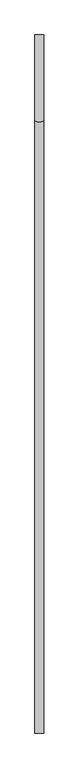
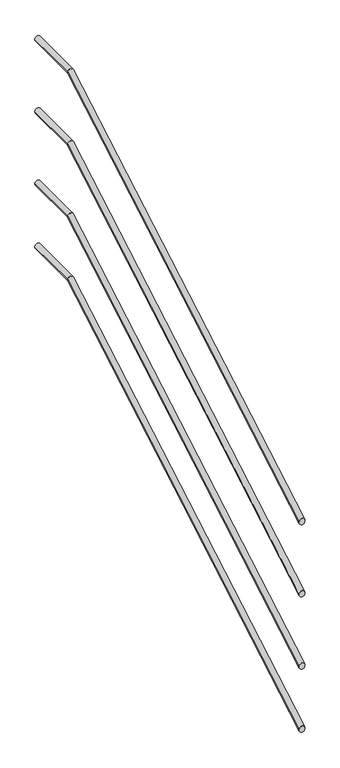
"""IFC4 building model written with IfcOpenShell, lengths in millimetres: railing geometry."""

import ifcopenshell
import ifcopenshell.guid

model = None  # the IFC model being written
_history = None  # IfcOwnerHistory: only IFC2X3 demands one
_inside = {}  # id of a spatial element -> (the spatial element, [elements in it])
_under = {}  # id of a project, library or spatial element -> (it, [spatial elements below it])
_declared = {}  # id of a project -> (the project, [libraries it declares])
_typed = {}  # id of a type object -> (the type object, [elements of that type])
_made_of = {}  # id of a material, layer set ... -> (it, [elements and type objects made of it])


def new_model(schema):
    """Start an empty IFC model of exactly this schema.

    Asked for "IFC4X3", IfcOpenShell would pick the latest addendum, in which some entities
    have other attributes; the version numbers below select the first issue.
    IFC2X3 requires an IfcOwnerHistory on every rooted entity: one is made here for all.
    """
    global model, _history
    if schema == "IFC4X3":
        model = ifcopenshell.file(schema_version=(4, 3, 0, 0))
    else:
        model = ifcopenshell.file(schema=schema)
    _inside.clear()
    _under.clear()
    _declared.clear()
    _typed.clear()
    _made_of.clear()
    _history = None
    if model.schema == "IFC2X3":
        org = make("IfcOrganization", Name="unknown")
        user = make(
            "IfcPersonAndOrganization",
            ThePerson=make("IfcPerson", FamilyName="unknown"),
            TheOrganization=org,
        )
        app = make(
            "IfcApplication",
            ApplicationDeveloper=org,
            Version="unknown",
            ApplicationFullName="unknown",
            ApplicationIdentifier="unknown",
        )
        _history = make(
            "IfcOwnerHistory",
            OwningUser=user,
            OwningApplication=app,
            ChangeAction="ADDED",
            CreationDate=0,
        )
    return model


def make(cls, **values):
    """One entity of the class cls with the attributes given. An attribute that is None is left unset."""
    return model.create_entity(
        cls, **{name: value for name, value in values.items() if value is not None}
    )


def rooted(cls, **values):
    """An entity with a GlobalId (a new one), such as an element, a storey or a relation."""
    return make(cls, GlobalId=ifcopenshell.guid.new(), OwnerHistory=_history, **values)


def si_unit(unit_type, name, prefix=None):
    """IfcSIUnit, for example si_unit("LENGTHUNIT", "METRE", prefix="MILLI")."""
    return make("IfcSIUnit", UnitType=unit_type, Prefix=prefix, Name=name)


def assignment(units):
    """IfcUnitAssignment: the units of a project."""
    return None if units is None else make("IfcUnitAssignment", Units=units)


def point(xyz):
    """IfcCartesianPoint."""
    return None if xyz is None else make("IfcCartesianPoint", Coordinates=xyz)


def direction(xyz):
    """IfcDirection."""
    return None if xyz is None else make("IfcDirection", DirectionRatios=xyz)


def frame(location, z_axis=None, x_axis=None):
    """IfcAxis2Placement3D, a coordinate frame: its origin and axes. An axis left out is left unset."""
    return make(
        "IfcAxis2Placement3D",
        Location=point(location),
        Axis=direction(z_axis),
        RefDirection=direction(x_axis),
    )


def origin():
    """The frame at (0, 0, 0) with its axes left unset."""
    return frame((0.0, 0.0, 0.0))


def place(relative_to, where):
    """IfcLocalPlacement: puts the frame where relative to a parent placement (None: the world)."""
    return make(
        "IfcLocalPlacement", PlacementRelTo=relative_to, RelativePlacement=where
    )


def context(
    kind, dimensions, precision=None, world=None, true_north=None, identifier=None
):
    """IfcGeometricRepresentationContext, for example the 3D "Model" context."""
    return make(
        "IfcGeometricRepresentationContext",
        ContextIdentifier=identifier,
        ContextType=kind,
        CoordinateSpaceDimension=dimensions,
        Precision=precision,
        WorldCoordinateSystem=world,
        TrueNorth=true_north,
    )


def project(units=None, contexts=None):
    """IfcProject with its units and contexts."""
    return rooted(
        "IfcProject",
        Name="project",
        RepresentationContexts=contexts,
        UnitsInContext=assignment(units),
    )


def spatial(cls, under=None, at=None, **own):
    """A site, building, storey or space (cls), placed at a placement, below another one or the project."""
    s = rooted(cls, ObjectPlacement=at, **own)
    if under is not None:
        _under.setdefault(under.id(), (under, []))[1].append(s)
    return s


def circle_curve(where, radius):
    """IfcCircle in the frame where."""
    return make("IfcCircle", Position=where, Radius=radius)


def ellipse_curve(where, semi_axis1, semi_axis2):
    """IfcEllipse in the frame where."""
    return make(
        "IfcEllipse", Position=where, SemiAxis1=semi_axis1, SemiAxis2=semi_axis2
    )


def shape(context_of_items, identifier, shape_type, items):
    """IfcShapeRepresentation: the items that make up one representation, for example the "Body"."""
    return make(
        "IfcShapeRepresentation",
        ContextOfItems=context_of_items,
        RepresentationIdentifier=identifier,
        RepresentationType=shape_type,
        Items=items,
    )


def source(mapping_origin, context_of_items, identifier, shape_type, items):
    """IfcRepresentationMap: a shape defined once, which mapped items show again and again."""
    return make(
        "IfcRepresentationMap",
        MappingOrigin=mapping_origin,
        MappedRepresentation=shape(context_of_items, identifier, shape_type, items),
    )


def transform(
    local_origin,
    x_axis=None,
    y_axis=None,
    z_axis=None,
    scale=None,
    scale2=None,
    scale3=None,
    uniform=True,
):
    """IfcCartesianTransformationOperator3D, or its non-uniform kind. x_axis, y_axis, z_axis: its Axis1, 2, 3."""
    if uniform:
        return make(
            "IfcCartesianTransformationOperator3D",
            Axis1=direction(x_axis),
            Axis2=direction(y_axis),
            LocalOrigin=point(local_origin),
            Scale=scale,
            Axis3=direction(z_axis),
        )
    return make(
        "IfcCartesianTransformationOperator3DnonUniform",
        Axis1=direction(x_axis),
        Axis2=direction(y_axis),
        LocalOrigin=point(local_origin),
        Scale=scale,
        Axis3=direction(z_axis),
        Scale2=scale2,
        Scale3=scale3,
    )


def mapped(mapping_source, mapping_target):
    """IfcMappedItem: shows the shape of a source again, moved by a transform."""
    return make(
        "IfcMappedItem", MappingSource=mapping_source, MappingTarget=mapping_target
    )


def made_of(thing, what):
    """Note that an element or type object is made of a material, layer set ...; save() writes the relation."""
    if what is not None:
        _made_of.setdefault(what.id(), (what, []))[1].append(thing)
    return thing


def element(
    cls,
    number,
    at=None,
    inside=None,
    cuts=None,
    type_object=None,
    material=None,
    context=None,
    identifier="Body",
    shape_type=None,
    held_by="IfcProductDefinitionShape",
    body=None,
    shapes=None,
    **own,
):
    """One element of the class cls, such as IfcWall. Its Tag is "e" and its number.

    at: its placement. inside: the storey or other place that contains it. cuts: it is an
    opening in that element (IfcRelVoidsElement). A single representation is given by context,
    identifier, shape_type and body (its items); several are given by shapes. held_by: the class
    of the entity that holds the representations. save() writes the other relations.
    """
    e = rooted(cls, Tag="e%d" % number, ObjectPlacement=at, **own)
    if body is not None:
        shapes = [shape(context, identifier, shape_type, body)]
    if shapes is not None:
        e.Representation = make(held_by, Representations=shapes)
    if inside is not None:
        _inside.setdefault(inside.id(), (inside, []))[1].append(e)
    if cuts is not None:
        rooted(
            "IfcRelVoidsElement", RelatingBuildingElement=cuts, RelatedOpeningElement=e
        )
    if type_object is not None:
        _typed.setdefault(type_object.id(), (type_object, []))[1].append(e)
    return made_of(e, material)


def aggregate(whole, parts):
    """IfcRelAggregates: a whole, such as a stair, and the parts it consists of."""
    return rooted("IfcRelAggregates", RelatingObject=whole, RelatedObjects=parts)


def save(model, path):
    """Write the relations noted so far, then the file.

    IfcRelAggregates (storeys below a building ...), IfcRelContainedInSpatialStructure (elements
    in a storey), IfcRelDefinesByType, IfcRelAssociatesMaterial and IfcRelDeclares: one each for
    every whole, place, type object, material and project.
    """
    for whole, parts in _under.values():
        aggregate(whole, parts)
    for where, things in _inside.values():
        rooted(
            "IfcRelContainedInSpatialStructure",
            RelatedElements=things,
            RelatingStructure=where,
        )
    for kind, things in _typed.values():
        rooted("IfcRelDefinesByType", RelatedObjects=things, RelatingType=kind)
    for what, things in _made_of.values():
        rooted("IfcRelAssociatesMaterial", RelatedObjects=things, RelatingMaterial=what)
    for by, libraries in _declared.values():
        rooted("IfcRelDeclares", RelatingContext=by, RelatedDefinitions=libraries)
    model.write(path)


def plane_surface(at):
    """IfcPlane: the flat surface through the origin of the frame at, square to its z axis."""
    return make("IfcPlane", Position=at)


def cylinder_surface(at, radius):
    """IfcCylindricalSurface: all points at the distance radius from the z axis of the frame at."""
    return make("IfcCylindricalSurface", Position=at, Radius=radius)


def advanced_brep(points, edges, surfaces, faces):
    """IfcAdvancedBrep: a solid bounded by faces that lie on surfaces and meet in shared edges.

    An edge is (start, end): straight between two places in points (the first is 0);
    or (start, end, curve); or (start, end, curve, False) where it runs against its curve.
    A face is (place in surfaces, loops), or (place, loops, False) where it looks against
    its surface's normal. A loop lists edges by number (the first is 1), with a minus sign
    where the edge is run from its end to its start. The first loop is the outer one.
    """
    corners = [point(p) for p in points]
    vertices = [make("IfcVertexPoint", VertexGeometry=c) for c in corners]
    made = []
    for start, end, *more in edges:
        made.append(
            make(
                "IfcEdgeCurve",
                EdgeStart=vertices[start],
                EdgeEnd=vertices[end],
                EdgeGeometry=more[0] if more else make("IfcPolyline", Points=[corners[start], corners[end]]),
                SameSense=more[1] if len(more) > 1 else True,
            )
        )
    hull = []
    for where, loops, *sense in faces:
        bounds = []
        for j, loop in enumerate(loops):
            ring = [make("IfcOrientedEdge", EdgeElement=made[abs(k) - 1], Orientation=k > 0) for k in loop]
            bounds.append(
                make(
                    "IfcFaceOuterBound" if j == 0 else "IfcFaceBound",
                    Bound=make("IfcEdgeLoop", EdgeList=ring),
                    Orientation=True,
                )
            )
        hull.append(make("IfcAdvancedFace", Bounds=bounds, FaceSurface=surfaces[where], SameSense=sense[0] if sense else True))
    return make("IfcAdvancedBrep", Outer=make("IfcClosedShell", CfsFaces=hull))


def railing_984455d7(model_context):
    return source(origin(), model_context, "Body", "AdvancedBrep", [
        advanced_brep(
        [(-1890.4, 13399.5208589, 4296.7361432), (-1860.4, 13399.5208589, 4296.7361432), (-1890.4, 15503.5584173, 5517.9030398), (-1860.4, 15503.5584173, 5517.9030398), (-1890.4, 15799.5208589, 5517.9030398), (-1860.4, 15799.5208589, 5517.9030398)],
        [
            (0, 1, ellipse_curve(frame((-1875.4, 13399.5208589, 4296.7361432), z_axis=(0.0, -1.0, 0.0), x_axis=(0.0, 0.0, -1.0)), 17.3433672, 15.0)),
            (1, 0, ellipse_curve(frame((-1875.4, 13399.5208589, 4296.7361432), z_axis=(0.0, -1.0, 0.0), x_axis=(0.0, 0.0, -1.0)), 17.3433672, 15.0)),
            (0, 2),
            (2, 3, ellipse_curve(frame((-1875.4, 15503.5584173, 5517.9030398), z_axis=(0.0, -0.9656303515230847, -0.2599192648062162), x_axis=(0.0, 0.2599192648062171, -0.9656303515230844)), 15.5338945, 15.0)),
            (3, 1),
            (3, 2, ellipse_curve(frame((-1875.4, 15503.5584173, 5517.9030398), z_axis=(0.0, -0.9656303515230847, -0.2599192648062162), x_axis=(0.0, 0.2599192648062171, -0.9656303515230844)), 15.5338945, 15.0)),
            (4, 5, circle_curve(frame((-1875.4, 15799.5208589, 5517.9030398), z_axis=(0.0, 1.0, 0.0), x_axis=(1.0, 0.0, 0.0)), 15.0)),
            (5, 4, circle_curve(frame((-1875.4, 15799.5208589, 5517.9030398), z_axis=(0.0, 1.0, 0.0), x_axis=(1.0, 0.0, 0.0)), 15.0)),
            (2, 4),
            (5, 3),
        ],
        [
            plane_surface(frame((-1875.4, 13399.5208589, 4314.0795104), z_axis=(0.0, -1.0, 0.0), x_axis=(0.0, 0.0, 1.0))),
            cylinder_surface(frame((-1875.4, 13407.0504368, 4301.1062512), z_axis=(0.0, -0.8648839515651922, -0.5019718620848966), x_axis=(1.0, 0.0, 0.0)), 15.0),
            plane_surface(frame((-1875.4, 15799.5208589, 5532.9030398), z_axis=(0.0, 1.0, 0.0), x_axis=(0.0, 0.0, 1.0))),
            cylinder_surface(frame((-1875.4, 15499.5208589, 5517.9030398), z_axis=(0.0, -1.0, 0.0), x_axis=(1.0, 0.0, 0.0)), 15.0),
        ],
        [
            (0, [[1, 2]]),
            (1, [[-1, 3, 4, 5]]),
            (1, [[-2, -5, 6, -3]]),
            (2, [[7, 8]]),
            (3, [[-4, 9, -8, 10]]),
            (3, [[-6, -10, -7, -9]]),
        ],
    ),
        advanced_brep(
        [(-1890.4, 13399.5208589, 3496.7361432), (-1860.4, 13399.5208589, 3496.7361432), (-1890.4, 15503.5584173, 4717.9030398), (-1860.4, 15503.5584173, 4717.9030398), (-1890.4, 15799.5208589, 4717.9030398), (-1860.4, 15799.5208589, 4717.9030398)],
        [
            (0, 1, ellipse_curve(frame((-1875.4, 13399.5208589, 3496.7361432), z_axis=(0.0, -1.0, 0.0), x_axis=(0.0, 0.0, -1.0)), 17.3433672, 15.0)),
            (1, 0, ellipse_curve(frame((-1875.4, 13399.5208589, 3496.7361432), z_axis=(0.0, -1.0, 0.0), x_axis=(0.0, 0.0, -1.0)), 17.3433672, 15.0)),
            (0, 2),
            (2, 3, ellipse_curve(frame((-1875.4, 15503.5584173, 4717.9030398), z_axis=(0.0, -0.9656303515230847, -0.2599192648062162), x_axis=(0.0, 0.2599192648062171, -0.9656303515230844)), 15.5338945, 15.0)),
            (3, 1),
            (3, 2, ellipse_curve(frame((-1875.4, 15503.5584173, 4717.9030398), z_axis=(0.0, -0.9656303515230847, -0.2599192648062162), x_axis=(0.0, 0.2599192648062171, -0.9656303515230844)), 15.5338945, 15.0)),
            (4, 5, circle_curve(frame((-1875.4, 15799.5208589, 4717.9030398), z_axis=(0.0, 1.0, 0.0), x_axis=(1.0, 0.0, 0.0)), 15.0)),
            (5, 4, circle_curve(frame((-1875.4, 15799.5208589, 4717.9030398), z_axis=(0.0, 1.0, 0.0), x_axis=(1.0, 0.0, 0.0)), 15.0)),
            (2, 4),
            (5, 3),
        ],
        [
            plane_surface(frame((-1875.4, 13399.5208589, 3514.0795104), z_axis=(0.0, -1.0, 0.0), x_axis=(0.0, 0.0, 1.0))),
            cylinder_surface(frame((-1875.4, 13407.0504368, 3501.1062512), z_axis=(0.0, -0.8648839515651922, -0.5019718620848966), x_axis=(1.0, 0.0, 0.0)), 15.0),
            plane_surface(frame((-1875.4, 15799.5208589, 4732.9030398), z_axis=(0.0, 1.0, 0.0), x_axis=(0.0, 0.0, 1.0))),
            cylinder_surface(frame((-1875.4, 15499.5208589, 4717.9030398), z_axis=(0.0, -1.0, 0.0), x_axis=(1.0, 0.0, 0.0)), 15.0),
        ],
        [
            (0, [[1, 2]]),
            (1, [[-1, 3, 4, 5]]),
            (1, [[-2, -5, 6, -3]]),
            (2, [[7, 8]]),
            (3, [[-4, 9, -8, 10]]),
            (3, [[-6, -10, -7, -9]]),
        ],
    ),
        advanced_brep(
        [(-1890.4, 13399.5208589, 3896.7361432), (-1860.4, 13399.5208589, 3896.7361432), (-1890.4, 15503.5584173, 5117.9030398), (-1860.4, 15503.5584173, 5117.9030398), (-1890.4, 15799.5208589, 5117.9030398), (-1860.4, 15799.5208589, 5117.9030398)],
        [
            (0, 1, ellipse_curve(frame((-1875.4, 13399.5208589, 3896.7361432), z_axis=(0.0, -1.0, 0.0), x_axis=(0.0, 0.0, -1.0)), 17.3433672, 15.0)),
            (1, 0, ellipse_curve(frame((-1875.4, 13399.5208589, 3896.7361432), z_axis=(0.0, -1.0, 0.0), x_axis=(0.0, 0.0, -1.0)), 17.3433672, 15.0)),
            (0, 2),
            (2, 3, ellipse_curve(frame((-1875.4, 15503.5584173, 5117.9030398), z_axis=(0.0, -0.9656303515230847, -0.2599192648062162), x_axis=(0.0, 0.2599192648062171, -0.9656303515230844)), 15.5338945, 15.0)),
            (3, 1),
            (3, 2, ellipse_curve(frame((-1875.4, 15503.5584173, 5117.9030398), z_axis=(0.0, -0.9656303515230847, -0.2599192648062162), x_axis=(0.0, 0.2599192648062171, -0.9656303515230844)), 15.5338945, 15.0)),
            (4, 5, circle_curve(frame((-1875.4, 15799.5208589, 5117.9030398), z_axis=(0.0, 1.0, 0.0), x_axis=(1.0, 0.0, 0.0)), 15.0)),
            (5, 4, circle_curve(frame((-1875.4, 15799.5208589, 5117.9030398), z_axis=(0.0, 1.0, 0.0), x_axis=(1.0, 0.0, 0.0)), 15.0)),
            (2, 4),
            (5, 3),
        ],
        [
            plane_surface(frame((-1875.4, 13399.5208589, 3914.0795104), z_axis=(0.0, -1.0, 0.0), x_axis=(0.0, 0.0, 1.0))),
            cylinder_surface(frame((-1875.4, 13407.0504368, 3901.1062512), z_axis=(0.0, -0.8648839515651922, -0.5019718620848966), x_axis=(1.0, 0.0, 0.0)), 15.0),
            plane_surface(frame((-1875.4, 15799.5208589, 5132.9030398), z_axis=(0.0, 1.0, 0.0), x_axis=(0.0, 0.0, 1.0))),
            cylinder_surface(frame((-1875.4, 15499.5208589, 5117.9030398), z_axis=(0.0, -1.0, 0.0), x_axis=(1.0, 0.0, 0.0)), 15.0),
        ],
        [
            (0, [[1, 2]]),
            (1, [[-1, 3, 4, 5]]),
            (1, [[-2, -5, 6, -3]]),
            (2, [[7, 8]]),
            (3, [[-4, 9, -8, 10]]),
            (3, [[-6, -10, -7, -9]]),
        ],
    ),
        advanced_brep(
        [(-1890.4, 13399.5208589, 3146.7361432), (-1860.4, 13399.5208589, 3146.7361432), (-1890.4, 15503.5584173, 4367.9030398), (-1860.4, 15503.5584173, 4367.9030398), (-1890.4, 15799.5208589, 4367.9030398), (-1860.4, 15799.5208589, 4367.9030398)],
        [
            (0, 1, ellipse_curve(frame((-1875.4, 13399.5208589, 3146.7361432), z_axis=(0.0, -1.0, 0.0), x_axis=(0.0, 0.0, -1.0)), 17.3433672, 15.0)),
            (1, 0, ellipse_curve(frame((-1875.4, 13399.5208589, 3146.7361432), z_axis=(0.0, -1.0, 0.0), x_axis=(0.0, 0.0, -1.0)), 17.3433672, 15.0)),
            (0, 2),
            (2, 3, ellipse_curve(frame((-1875.4, 15503.5584173, 4367.9030398), z_axis=(0.0, -0.9656303515230847, -0.2599192648062162), x_axis=(0.0, 0.2599192648062171, -0.9656303515230844)), 15.5338945, 15.0)),
            (3, 1),
            (3, 2, ellipse_curve(frame((-1875.4, 15503.5584173, 4367.9030398), z_axis=(0.0, -0.9656303515230847, -0.2599192648062162), x_axis=(0.0, 0.2599192648062171, -0.9656303515230844)), 15.5338945, 15.0)),
            (4, 5, circle_curve(frame((-1875.4, 15799.5208589, 4367.9030398), z_axis=(0.0, 1.0, 0.0), x_axis=(1.0, 0.0, 0.0)), 15.0)),
            (5, 4, circle_curve(frame((-1875.4, 15799.5208589, 4367.9030398), z_axis=(0.0, 1.0, 0.0), x_axis=(1.0, 0.0, 0.0)), 15.0)),
            (2, 4),
            (5, 3),
        ],
        [
            plane_surface(frame((-1875.4, 13399.5208589, 3164.0795104), z_axis=(0.0, -1.0, 0.0), x_axis=(0.0, 0.0, 1.0))),
            cylinder_surface(frame((-1875.4, 13407.0504368, 3151.1062512), z_axis=(0.0, -0.8648839515651922, -0.5019718620848966), x_axis=(1.0, 0.0, 0.0)), 15.0),
            plane_surface(frame((-1875.4, 15799.5208589, 4382.9030398), z_axis=(0.0, 1.0, 0.0), x_axis=(0.0, 0.0, 1.0))),
            cylinder_surface(frame((-1875.4, 15499.5208589, 4367.9030398), z_axis=(0.0, -1.0, 0.0), x_axis=(1.0, 0.0, 0.0)), 15.0),
        ],
        [
            (0, [[1, 2]]),
            (1, [[-1, 3, 4, 5]]),
            (1, [[-2, -5, 6, -3]]),
            (2, [[7, 8]]),
            (3, [[-4, 9, -8, 10]]),
            (3, [[-6, -10, -7, -9]]),
        ],
    ),
    ])


if __name__ == "__main__":
    model = new_model("IFC4")
    model_context = context("Model", 3, world=origin())
    ifc_project = project(units=[si_unit("LENGTHUNIT", "METRE", prefix="MILLI")], contexts=[model_context])
    site = spatial("IfcSite", under=ifc_project)
    building = spatial("IfcBuilding", under=site)
    placement = place(None, origin())
    railing_shape = railing_984455d7(model_context)
    element("IfcRailing", 1, at=placement, inside=building, context=model_context, shape_type="MappedRepresentation", body=[
        mapped(railing_shape, transform((0.0, 0.0, 0.0), x_axis=(1.0, 0.0, 0.0), y_axis=(0.0, 1.0, 0.0), z_axis=(0.0, 0.0, 1.0))),
    ])
    save(model, "model.ifc")
